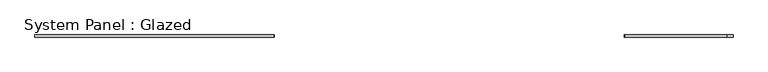
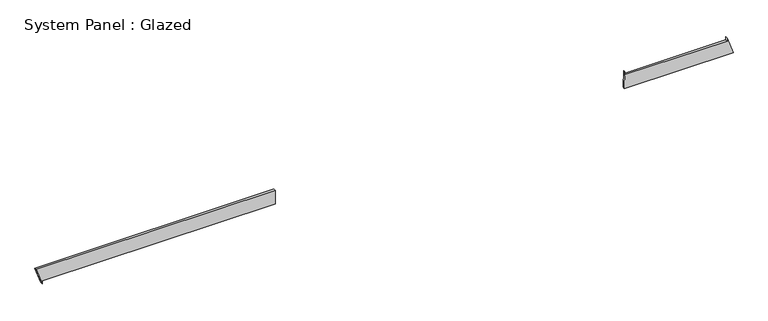
"""IFC4 building model written with IfcOpenShell, lengths in millimetres: plate geometry, System Panel : Glazed."""

from ifc_helpers import new_model, si_unit, frame, origin, place, context, project, spatial, polyline, outline, extrude, source, transform, mapped, element, save


def system_panel_glazed_c0dc2f60(model_context):
    return source(origin(), model_context, "Body", "SweptSolid", [
        extrude(outline(polyline([(35.3553391, 2769.8232557), (35.3553391, 4027.0933919), (235.3468796, 3957.4323455), (199.9915406, 3957.4328486), (199.9747344, 2776.4489801), (235.3300734, 2776.448477), (35.3553391, 2769.8232557)])), frame((0.0, -49.5, 0.0), z_axis=(0.0, 1.0, 0.0), x_axis=(0.0, 0.0, 1.0)), (0.0, 0.0, 1.0), 25.0),
        extrude(outline(polyline([(0.0, -3957.1612499), (35.3553391, -3957.1612499), (35.3553391, -1263.2772426), (199.9172113, -1265.7383879), (199.8779154, -4027.0933919), (0.0, -3957.1612499)])), frame((0.0, -49.5, 0.0), z_axis=(0.0, 1.0, 0.0), x_axis=(0.0, 0.0, 1.0)), (0.0, 0.0, 1.0), 25.0),
    ])


if __name__ == "__main__":
    model = new_model("IFC4")
    model_context = context("Model", 3, world=origin())
    ifc_project = project(units=[si_unit("LENGTHUNIT", "METRE", prefix="MILLI")], contexts=[model_context])
    site = spatial("IfcSite", under=ifc_project)
    building = spatial("IfcBuilding", under=site)
    placement = place(None, origin())
    system_panel_glazed_shape = system_panel_glazed_c0dc2f60(model_context)
    element("IfcPlate", 1, ObjectType="System Panel : Glazed", at=placement, inside=building, context=model_context, shape_type="MappedRepresentation", body=[
        mapped(system_panel_glazed_shape, transform((0.0, 0.0, 0.0), x_axis=(1.0, 0.0, 0.0), y_axis=(0.0, 1.0, 0.0), z_axis=(0.0, 0.0, 1.0))),
    ])
    save(model, "model.ifc")

# Revit data of these elements
# Element 1 (IfcPlate, "System Panel : Glazed")
#   Materials on its faces: "Glass"
# Materials
#   "Glass": class "Glass", colour RGB 218 227 224, transparency 0.85, Description = "Soda Lime Glass", Cost = 0
